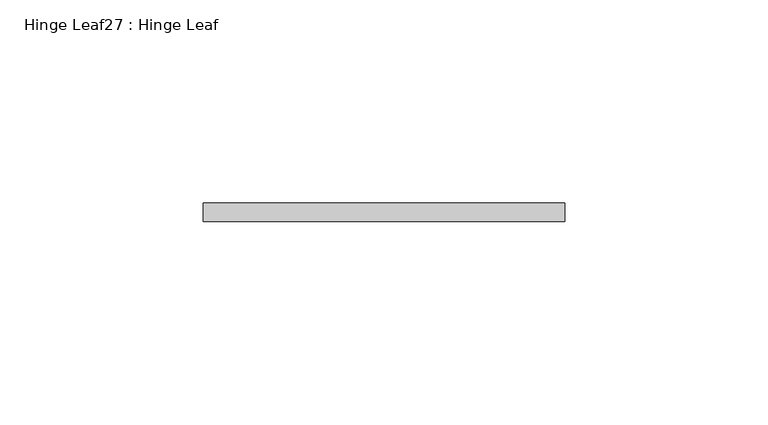
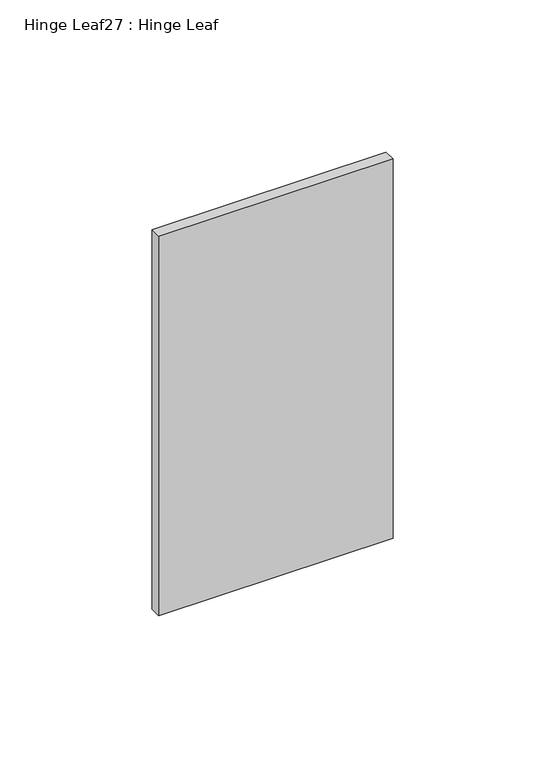
"""IFC4 building model written with IfcOpenShell, lengths in millimetres: proxy geometry, Hinge Leaf27 : Hinge Leaf."""

from ifc_helpers import new_model, si_unit, frame, origin, place, context, project, spatial, polyline, outline, extrude, source, transform, mapped, element, save


def hinge_leaf27_hinge_leaf_4683ff22(model_context):
    return source(origin(), model_context, "Body", "SweptSolid", [
        extrude(outline(polyline([(587327.7934739, -531772.5663841), (587416.6934739, -531772.5663841), (587416.6934739, -531777.1383841), (587327.7934739, -531777.1383841), (587327.7934739, -531772.5663841)])), frame((0.0, 0.0, 311.15), z_axis=(0.0, 0.0, 1.0), x_axis=(1.0, 0.0, 0.0)), (0.0, 0.0, 1.0), 152.4),
    ])


if __name__ == "__main__":
    model = new_model("IFC4")
    model_context = context("Model", 3, world=origin())
    ifc_project = project(units=[si_unit("LENGTHUNIT", "METRE", prefix="MILLI")], contexts=[model_context])
    site = spatial("IfcSite", under=ifc_project)
    building = spatial("IfcBuilding", under=site)
    placement = place(None, origin())
    hinge_leaf27_hinge_leaf_shape = hinge_leaf27_hinge_leaf_4683ff22(model_context)
    element("IfcBuildingElementProxy", 1, Name="Hinge Leaf27 : Hinge Leaf", ObjectType="Hinge Leaf27 : Hinge Leaf", at=placement, inside=building, context=model_context, shape_type="MappedRepresentation", body=[
        mapped(hinge_leaf27_hinge_leaf_shape, transform((0.0, 0.0, 0.0), x_axis=(1.0, 0.0, 0.0), y_axis=(0.0, 1.0, 0.0), z_axis=(0.0, 0.0, 1.0))),
    ])
    save(model, "model.ifc")

# Revit data of these elements
# Element 1 (IfcBuildingElementProxy, "Hinge Leaf27 : Hinge Leaf")
#   Materials on its faces: "6\"X6\" WELD-ON STL BUTT HINGE"
# Materials
#   "6\"X6\" WELD-ON STL BUTT HINGE": class "Metal", colour RGB 189 187 185, transparency 0, Description = "Carbon steel", Cost = 0
